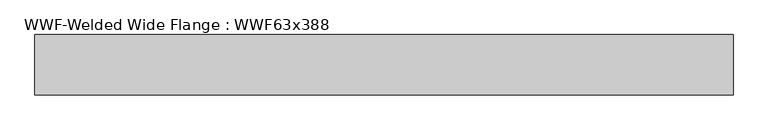
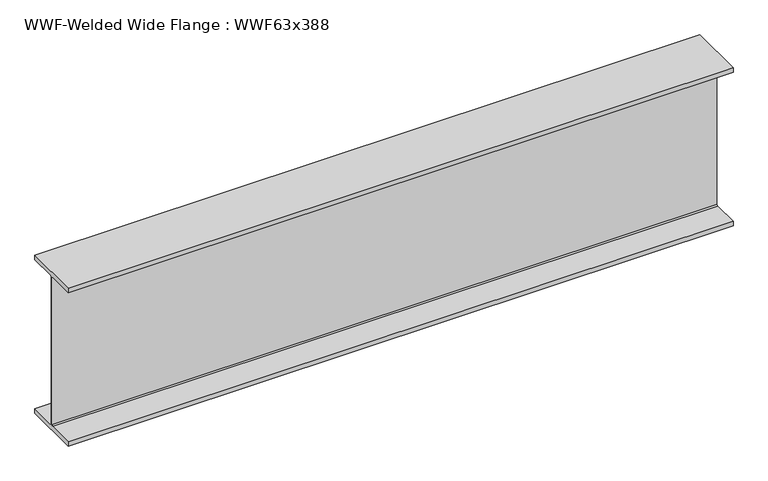
"""IFC4 building model written with IfcOpenShell, lengths in millimetres: beam geometry, WWF-Welded Wide Flange : WWF63x388."""

from ifc_helpers import new_model, si_unit, frame, origin, place, context, project, spatial, polyline, outline, extrude, source, transform, mapped, element, save


def wwf_welded_wide_flange_wwf63x388_8b89d44d(model_context):
    return source(origin(), model_context, "Body", "SweptSolid", [
        extrude(outline(polyline([(274.955, -755.015), (274.955, -799.973), (-274.955, -799.973), (-274.955, -755.015), (-19.05, -755.015), (-8.001, -743.966), (-8.001, 743.966), (-19.05, 755.015), (-274.955, 755.015), (-274.955, 799.973), (274.955, 799.973), (274.955, 755.015), (19.05, 755.015), (8.001, 743.966), (8.001, -743.966), (19.05, -755.015), (274.955, -755.015)])), frame((-3184.5866542, 0.0, 0.0), z_axis=(1.0, 0.0, 0.0), x_axis=(0.0, 1.0, 0.0)), (0.0, 0.0, 1.0), 6369.1344444),
    ])


if __name__ == "__main__":
    model = new_model("IFC4")
    model_context = context("Model", 3, world=origin())
    ifc_project = project(units=[si_unit("LENGTHUNIT", "METRE", prefix="MILLI")], contexts=[model_context])
    site = spatial("IfcSite", under=ifc_project)
    building = spatial("IfcBuilding", under=site)
    placement = place(None, origin())
    wwf_welded_wide_flange_wwf63x388_shape = wwf_welded_wide_flange_wwf63x388_8b89d44d(model_context)
    element("IfcBeam", 1, ObjectType="WWF-Welded Wide Flange : WWF63x388", at=placement, inside=building, context=model_context, shape_type="MappedRepresentation", body=[
        mapped(wwf_welded_wide_flange_wwf63x388_shape, transform((0.0, 0.0, 0.0), x_axis=(1.0, 0.0, 0.0), y_axis=(0.0, 1.0, 0.0), z_axis=(0.0, 0.0, 1.0))),
    ])
    save(model, "model.ifc")

# Revit data of these elements
# Type "WWF-Welded Wide Flange : WWF63x388"
#   Assembly Code = "B10"
#   Nominal d = "12"
#   W = 388
#   Length [instance default] = 1524 mm
#   bf = 549.91 mm
#   d = 1599.946 mm
#   k = 19.05 mm
#   tf = 44.958 mm
#   tw = 16.002 mm
#   A = 0.0735482 m²
#   Structural Material [instance default] = Steel ASTM A572
# Element 1 (IfcBeam, "WWF-Welded Wide Flange : WWF63x388")
#   Structural Material = Metal - Steel 43-275
#   Materials on its faces: "Metal - Steel 43-275"
# Materials
#   "Steel ASTM A572": class "Metal", colour RGB 247 247 247, transparency 0, Description = "Structural steel, high strength low alloy, ASTM - A572 - 50", Cost = 0
#   "Metal - Steel 43-275": class "Metal", colour RGB 247 247 247, transparency 0, Cost = 0
